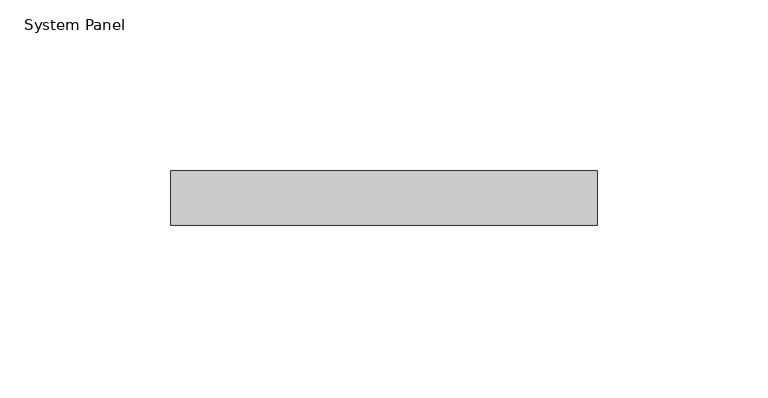
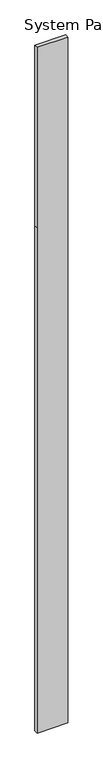
"""IFC4 building model written with IfcOpenShell, lengths in millimetres: plate geometry, System Panel : 로이복층유리_16."""

import ifcopenshell
import ifcopenshell.guid

model = None  # the IFC model being written
_history = None  # IfcOwnerHistory: only IFC2X3 demands one
_inside = {}  # id of a spatial element -> (the spatial element, [elements in it])
_under = {}  # id of a project, library or spatial element -> (it, [spatial elements below it])
_declared = {}  # id of a project -> (the project, [libraries it declares])
_typed = {}  # id of a type object -> (the type object, [elements of that type])
_made_of = {}  # id of a material, layer set ... -> (it, [elements and type objects made of it])


def new_model(schema):
    """Start an empty IFC model of exactly this schema.

    Asked for "IFC4X3", IfcOpenShell would pick the latest addendum, in which some entities
    have other attributes; the version numbers below select the first issue.
    IFC2X3 requires an IfcOwnerHistory on every rooted entity: one is made here for all.
    """
    global model, _history
    if schema == "IFC4X3":
        model = ifcopenshell.file(schema_version=(4, 3, 0, 0))
    else:
        model = ifcopenshell.file(schema=schema)
    _inside.clear()
    _under.clear()
    _declared.clear()
    _typed.clear()
    _made_of.clear()
    _history = None
    if model.schema == "IFC2X3":
        org = make("IfcOrganization", Name="unknown")
        user = make(
            "IfcPersonAndOrganization",
            ThePerson=make("IfcPerson", FamilyName="unknown"),
            TheOrganization=org,
        )
        app = make(
            "IfcApplication",
            ApplicationDeveloper=org,
            Version="unknown",
            ApplicationFullName="unknown",
            ApplicationIdentifier="unknown",
        )
        _history = make(
            "IfcOwnerHistory",
            OwningUser=user,
            OwningApplication=app,
            ChangeAction="ADDED",
            CreationDate=0,
        )
    return model


def make(cls, **values):
    """One entity of the class cls with the attributes given. An attribute that is None is left unset."""
    return model.create_entity(
        cls, **{name: value for name, value in values.items() if value is not None}
    )


def rooted(cls, **values):
    """An entity with a GlobalId (a new one), such as an element, a storey or a relation."""
    return make(cls, GlobalId=ifcopenshell.guid.new(), OwnerHistory=_history, **values)


def si_unit(unit_type, name, prefix=None):
    """IfcSIUnit, for example si_unit("LENGTHUNIT", "METRE", prefix="MILLI")."""
    return make("IfcSIUnit", UnitType=unit_type, Prefix=prefix, Name=name)


def assignment(units):
    """IfcUnitAssignment: the units of a project."""
    return None if units is None else make("IfcUnitAssignment", Units=units)


def point(xyz):
    """IfcCartesianPoint."""
    return None if xyz is None else make("IfcCartesianPoint", Coordinates=xyz)


def direction(xyz):
    """IfcDirection."""
    return None if xyz is None else make("IfcDirection", DirectionRatios=xyz)


def frame(location, z_axis=None, x_axis=None):
    """IfcAxis2Placement3D, a coordinate frame: its origin and axes. An axis left out is left unset."""
    return make(
        "IfcAxis2Placement3D",
        Location=point(location),
        Axis=direction(z_axis),
        RefDirection=direction(x_axis),
    )


def origin():
    """The frame at (0, 0, 0) with its axes left unset."""
    return frame((0.0, 0.0, 0.0))


def place(relative_to, where):
    """IfcLocalPlacement: puts the frame where relative to a parent placement (None: the world)."""
    return make(
        "IfcLocalPlacement", PlacementRelTo=relative_to, RelativePlacement=where
    )


def context(
    kind, dimensions, precision=None, world=None, true_north=None, identifier=None
):
    """IfcGeometricRepresentationContext, for example the 3D "Model" context."""
    return make(
        "IfcGeometricRepresentationContext",
        ContextIdentifier=identifier,
        ContextType=kind,
        CoordinateSpaceDimension=dimensions,
        Precision=precision,
        WorldCoordinateSystem=world,
        TrueNorth=true_north,
    )


def project(units=None, contexts=None):
    """IfcProject with its units and contexts."""
    return rooted(
        "IfcProject",
        Name="project",
        RepresentationContexts=contexts,
        UnitsInContext=assignment(units),
    )


def spatial(cls, under=None, at=None, **own):
    """A site, building, storey or space (cls), placed at a placement, below another one or the project."""
    s = rooted(cls, ObjectPlacement=at, **own)
    if under is not None:
        _under.setdefault(under.id(), (under, []))[1].append(s)
    return s


def polyline(points):
    """IfcPolyline through the points."""
    return make("IfcPolyline", Points=[point(p) for p in points])


def outline(outer, holes=None, kind="AREA"):
    """IfcArbitraryClosedProfileDef: a profile drawn as a closed curve; with holes, ...WithVoids."""
    if holes is None:
        return make("IfcArbitraryClosedProfileDef", ProfileType=kind, OuterCurve=outer)
    return make(
        "IfcArbitraryProfileDefWithVoids",
        ProfileType=kind,
        OuterCurve=outer,
        InnerCurves=holes,
    )


def extrude(swept, where, along, depth):
    """IfcExtrudedAreaSolid: the profile swept, set in the frame where, extruded along a direction by depth."""
    return make(
        "IfcExtrudedAreaSolid",
        SweptArea=swept,
        Position=where,
        ExtrudedDirection=direction(along),
        Depth=depth,
    )


def shape(context_of_items, identifier, shape_type, items):
    """IfcShapeRepresentation: the items that make up one representation, for example the "Body"."""
    return make(
        "IfcShapeRepresentation",
        ContextOfItems=context_of_items,
        RepresentationIdentifier=identifier,
        RepresentationType=shape_type,
        Items=items,
    )


def source(mapping_origin, context_of_items, identifier, shape_type, items):
    """IfcRepresentationMap: a shape defined once, which mapped items show again and again."""
    return make(
        "IfcRepresentationMap",
        MappingOrigin=mapping_origin,
        MappedRepresentation=shape(context_of_items, identifier, shape_type, items),
    )


def transform(
    local_origin,
    x_axis=None,
    y_axis=None,
    z_axis=None,
    scale=None,
    scale2=None,
    scale3=None,
    uniform=True,
):
    """IfcCartesianTransformationOperator3D, or its non-uniform kind. x_axis, y_axis, z_axis: its Axis1, 2, 3."""
    if uniform:
        return make(
            "IfcCartesianTransformationOperator3D",
            Axis1=direction(x_axis),
            Axis2=direction(y_axis),
            LocalOrigin=point(local_origin),
            Scale=scale,
            Axis3=direction(z_axis),
        )
    return make(
        "IfcCartesianTransformationOperator3DnonUniform",
        Axis1=direction(x_axis),
        Axis2=direction(y_axis),
        LocalOrigin=point(local_origin),
        Scale=scale,
        Axis3=direction(z_axis),
        Scale2=scale2,
        Scale3=scale3,
    )


def mapped(mapping_source, mapping_target):
    """IfcMappedItem: shows the shape of a source again, moved by a transform."""
    return make(
        "IfcMappedItem", MappingSource=mapping_source, MappingTarget=mapping_target
    )


def made_of(thing, what):
    """Note that an element or type object is made of a material, layer set ...; save() writes the relation."""
    if what is not None:
        _made_of.setdefault(what.id(), (what, []))[1].append(thing)
    return thing


def element(
    cls,
    number,
    at=None,
    inside=None,
    cuts=None,
    type_object=None,
    material=None,
    context=None,
    identifier="Body",
    shape_type=None,
    held_by="IfcProductDefinitionShape",
    body=None,
    shapes=None,
    **own,
):
    """One element of the class cls, such as IfcWall. Its Tag is "e" and its number.

    at: its placement. inside: the storey or other place that contains it. cuts: it is an
    opening in that element (IfcRelVoidsElement). A single representation is given by context,
    identifier, shape_type and body (its items); several are given by shapes. held_by: the class
    of the entity that holds the representations. save() writes the other relations.
    """
    e = rooted(cls, Tag="e%d" % number, ObjectPlacement=at, **own)
    if body is not None:
        shapes = [shape(context, identifier, shape_type, body)]
    if shapes is not None:
        e.Representation = make(held_by, Representations=shapes)
    if inside is not None:
        _inside.setdefault(inside.id(), (inside, []))[1].append(e)
    if cuts is not None:
        rooted(
            "IfcRelVoidsElement", RelatingBuildingElement=cuts, RelatedOpeningElement=e
        )
    if type_object is not None:
        _typed.setdefault(type_object.id(), (type_object, []))[1].append(e)
    return made_of(e, material)


def aggregate(whole, parts):
    """IfcRelAggregates: a whole, such as a stair, and the parts it consists of."""
    return rooted("IfcRelAggregates", RelatingObject=whole, RelatedObjects=parts)


def save(model, path):
    """Write the relations noted so far, then the file.

    IfcRelAggregates (storeys below a building ...), IfcRelContainedInSpatialStructure (elements
    in a storey), IfcRelDefinesByType, IfcRelAssociatesMaterial and IfcRelDeclares: one each for
    every whole, place, type object, material and project.
    """
    for whole, parts in _under.values():
        aggregate(whole, parts)
    for where, things in _inside.values():
        rooted(
            "IfcRelContainedInSpatialStructure",
            RelatedElements=things,
            RelatingStructure=where,
        )
    for kind, things in _typed.values():
        rooted("IfcRelDefinesByType", RelatedObjects=things, RelatingType=kind)
    for what, things in _made_of.values():
        rooted("IfcRelAssociatesMaterial", RelatedObjects=things, RelatingMaterial=what)
    for by, libraries in _declared.values():
        rooted("IfcRelDeclares", RelatingContext=by, RelatedDefinitions=libraries)
    model.write(path)


def system_panel_96f521d3(model_context):
    return source(origin(), model_context, "Body", "SweptSolid", [
        extrude(outline(polyline([(0.0, -62.5), (0.0, 62.5), (2177.5, 62.5), (2955.0, 62.5), (2955.0, -62.5), (2177.5, -62.5), (0.0, -62.5)])), frame((0.0, -8.0, 0.0), z_axis=(0.0, 1.0, 0.0), x_axis=(0.0, 0.0, 1.0)), (0.0, 0.0, 1.0), 16.0),
    ])


if __name__ == "__main__":
    model = new_model("IFC4")
    model_context = context("Model", 3, world=origin())
    ifc_project = project(units=[si_unit("LENGTHUNIT", "METRE", prefix="MILLI")], contexts=[model_context])
    site = spatial("IfcSite", under=ifc_project)
    building = spatial("IfcBuilding", under=site)
    placement = place(None, origin())
    system_panel_shape = system_panel_96f521d3(model_context)
    element("IfcPlate", 1, ObjectType="System Panel : 로이복층유리_16", at=placement, inside=building, context=model_context, shape_type="MappedRepresentation", body=[
        mapped(system_panel_shape, transform((0.0, 0.0, 0.0), x_axis=(1.0, 0.0, 0.0), y_axis=(0.0, 1.0, 0.0), z_axis=(0.0, 0.0, 1.0))),
    ])
    save(model, "model.ifc")

# Revit data of these elements
# Element 1 (IfcPlate, "System Panel : 로이복층유리_16")
#   Materials on its faces: "00_Glass_Glass"
# Materials
#   "00_Glass_Glass": class "Glass", colour RGB 218 227 224, transparency 0.85, Description = "Glass", Cost = 0, Image = none
